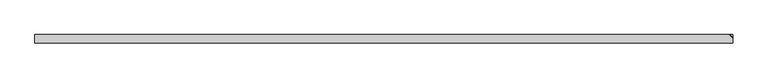
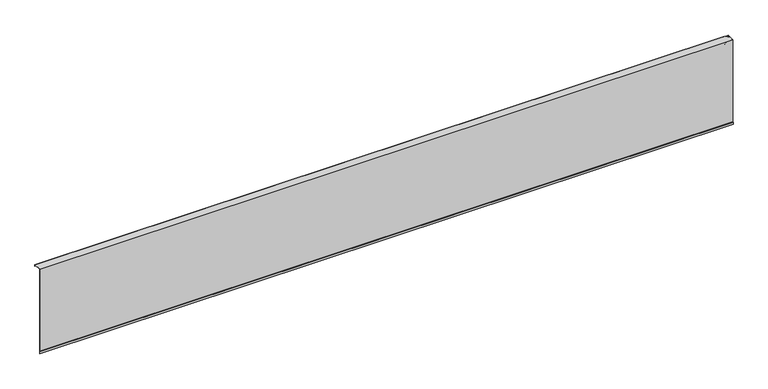
"""IFC4 building model written with IfcOpenShell, lengths in millimetres: proxy geometry, Generic Models 7:Generic Models 1:5:Generic Models 1:5 : Generic Models 7:Generic Models 1:337419:9 : Generic Models 7:Generic Models 1:5:Generic Models 1:5 : Generic Models 7:Generic Models 1:337419:311462."""

from ifc_helpers import new_model, si_unit, origin, place, context, project, spatial, faceted_brep, source, transform, mapped, element, save


def generic_models_b51a2378(model_context):
    return source(origin(), model_context, "Body", "Brep", [
        faceted_brep([(579322.7929739, -579015.7726341, 3809.9499966), (579322.7929739, -579026.4643504, 3794.6806432), (579322.7929739, -579026.4643504, 3735.8407393), (579322.7929739, -579024.8768504, 3735.8407393), (579322.7929739, -579024.8768504, 3794.1801063), (579322.7929739, -579014.1851341, 3809.4494597), (579322.7929739, -579014.1851341, 4170.3683016), (579322.7929739, -579015.7726341, 4170.3683016), (560352.1692831, -579014.1851341, 6179.105206), (560352.1692831, -579014.1851341, 3809.4494597), (560352.1692831, -579024.8768504, 3794.1801063), (560352.1692831, -579024.8768504, 3735.8407393), (560352.1692831, -579026.4643504, 3735.8407393), (560352.1692831, -579026.4643504, 3794.6806432), (560352.1692831, -579015.7726341, 3809.9499966), (560352.1692831, -579015.7726341, 6180.7780819), (560352.1692831, -578793.4990368, 6169.1292163), (560352.1692831, -578793.4990368, 6125.2823817), (560352.1692831, -578795.0865368, 6125.2823817), (560352.1692831, -578795.0865368, 6167.622735), (579321.2054739, -579015.7726341, 4172.6354866), (579321.2054739, -579015.7726341, 6172.5888113), (579102.1068767, -579015.7726341, 6161.1063403), (579102.1068767, -579015.7726341, 6125.115987), (579100.5193767, -579015.7726341, 6125.115987), (579100.5193767, -579015.7726341, 6162.6128216), (579322.7929739, -579015.7726341, 6174.2616872), (579322.7929739, -579015.7726341, 6180.7780819), (579322.7929739, -579014.1851341, 6179.105206), (579322.7929739, -579014.1851341, 6174.2616872), (579100.5193767, -579014.1851341, 6162.6128216), (579100.5193767, -579014.1851341, 6125.115987), (579102.1068767, -579014.1851341, 6125.115987), (579102.1068767, -579014.1851341, 6161.1063403), (579321.2054739, -579014.1851341, 6172.5888113), (579321.2054739, -579014.1851341, 4172.6354866), (579322.7929739, -578921.7652908, 6174.2616872), (579322.7929739, -578891.4324161, 6174.2616872), (579196.11422, -578795.0865368, 6167.622735), (579100.5193767, -578795.0865368, 6125.2823817), (579100.5193767, -578795.0865368, 6162.6128216), (579100.5193767, -578793.4990368, 6125.2823817), (579224.8595947, -578793.4990368, 6169.1292163), (579100.5193767, -578793.4990368, 6162.6128216)], [[[0, 1, 2, 3, 4, 5, 6, 7]], [[8, 9, 10, 11, 12, 13, 14, 15, 16, 17, 18, 19]], [[15, 14, 0, 7, 20, 21, 22, 23, 24, 25, 26, 27]], [[1, 0, 14, 13]], [[2, 1, 13, 12]], [[3, 2, 12, 11]], [[4, 3, 11, 10]], [[5, 4, 10, 9]], [[9, 8, 28, 29, 30, 31, 32, 33, 34, 35, 6, 5]], [[35, 20, 7, 6]], [[20, 35, 34, 21]], [[21, 34, 33, 22]], [[22, 33, 32, 23]], [[23, 32, 31, 24]], [[24, 31, 30, 25]], [[25, 30, 29, 26]], [[29, 28, 36, 37, 27, 26]], [[8, 19, 38, 36, 28]], [[19, 18, 39, 40, 38]], [[18, 17, 41, 39]], [[17, 16, 42, 43, 41]], [[16, 15, 27, 37, 42]], [[43, 40, 39, 41]], [[40, 43, 42, 37, 36, 38]]]),
        faceted_brep([(579226.4470947, -578795.0865368, 6167.622735), (579321.2054739, -578795.0865368, 6167.622735), (579321.2054739, -578889.8449161, 6172.5888113), (579102.1068767, -578795.0865368, 6161.1063403), (579102.1068767, -578795.0865368, 6125.2823817), (579321.2054739, -578795.0865368, 6125.2823817), (579102.1068767, -578793.4990368, 6125.2823817), (579321.2054739, -578793.4990368, 6125.2823817), (579102.1068767, -578793.4990368, 6161.1063403), (579255.1924693, -578793.4990368, 6169.1292163), (579321.2054739, -578793.4990368, 6169.1292163), (579321.2054739, -578859.5120415, 6172.5888113)], [[[0, 1, 2]], [[1, 0, 3, 4, 5]], [[5, 4, 6, 7]], [[7, 6, 8, 9, 10]], [[10, 9, 11]], [[11, 2, 1, 5, 7, 10]], [[2, 11, 9, 8, 3, 0]], [[3, 8, 6, 4]]]),
    ])


if __name__ == "__main__":
    model = new_model("IFC4")
    model_context = context("Model", 3, world=origin())
    ifc_project = project(units=[si_unit("LENGTHUNIT", "METRE", prefix="MILLI")], contexts=[model_context])
    site = spatial("IfcSite", under=ifc_project)
    building = spatial("IfcBuilding", under=site)
    placement = place(None, origin())
    generic_models_shape = generic_models_b51a2378(model_context)
    element("IfcBuildingElementProxy", 1, Name="Generic Models 7:Generic Models 1:5:Generic Models 1:5 : Generic Models 7:Generic Models 1:337419:9 : Generic Models 7:Generic Models 1:5:Generic Models 1:5 : Generic Models 7:Generic Models 1:337419:311462", ObjectType="Generic Models 7:Generic Models 1:5:Generic Models 1:5 : Generic Models 7:Generic Models 1:337419:9 : Generic Models 7:Generic Models 1:5:Generic Models 1:5 : Generic Models 7:Generic Models 1:337419:311462", at=placement, inside=building, context=model_context, shape_type="MappedRepresentation", body=[
        mapped(generic_models_shape, transform((0.0, 0.0, 0.0), x_axis=(1.0, 0.0, 0.0), y_axis=(0.0, 1.0, 0.0), z_axis=(0.0, 0.0, 1.0))),
    ])
    save(model, "model.ifc")

# Revit data of these elements
# Type "Generic Models 7:Generic Models 1:5:Generic Models 1:5 : Generic Models 7:Generic Models 1:337419:9 : Generic Models 7:Generic Models 1:5:Generic Models 1:5 : Generic Models 7:Generic Models 1:337419:311462"
#   NameOverride = "Generic Models 7:Generic Models 1:5:Generic Models 1:5 : Generic Models 7:Generic Models 1:337419:311462"
#   ObjectTypeOverride = "Generic Models 1:5 : Generic Models 7:Generic Models 1:337419"
#   Reference = "Generic Models 1"
#   Tag = "311462"
# Element 1 (IfcBuildingElementProxy, "Generic Models 7:Generic Models 1:5:Generic Models 1:5 : Generic Models 7:Generic Models 1:337419:9 : Generic Models 7:Generic Models 1:5:Generic Models 1:5 : Generic Models 7:Generic Models 1:337419:311462")
#   Materials on its faces: "UV STABLE WATER RESISTANT VAPOR PERMEABLE AIR BARRIER (WRB) - WRAP JAMBS/HEADERS - BLACK COLOR"
# Materials
#   "UV STABLE WATER RESISTANT VAPOR PERMEABLE AIR BARRIER (WRB) - WRAP JAMBS/HEADERS - BLACK COLOR": class "Generic", colour RGB 51 162 45, transparency 0, Description = "Polyethylene film membrane", Cost = 0
